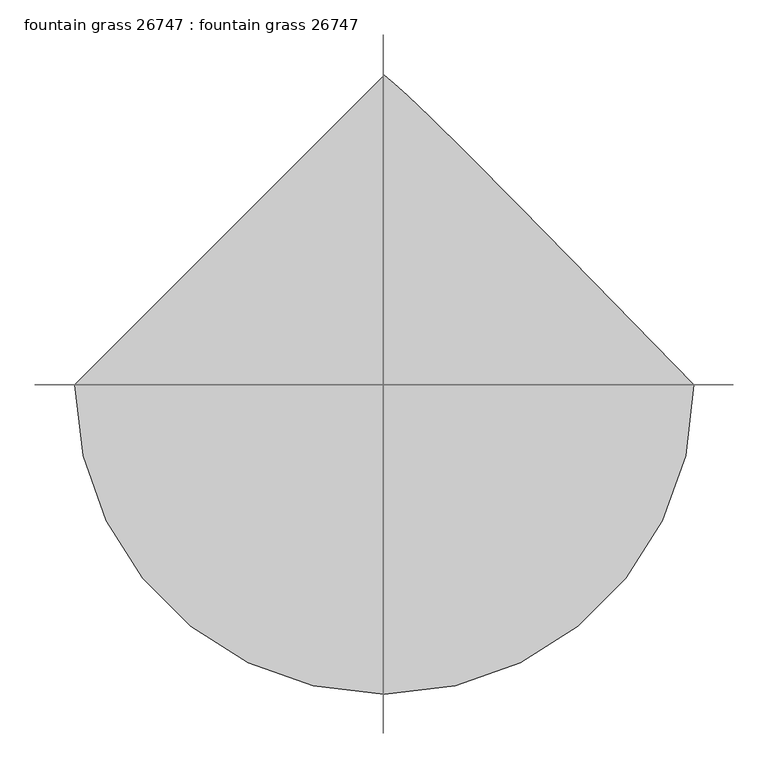
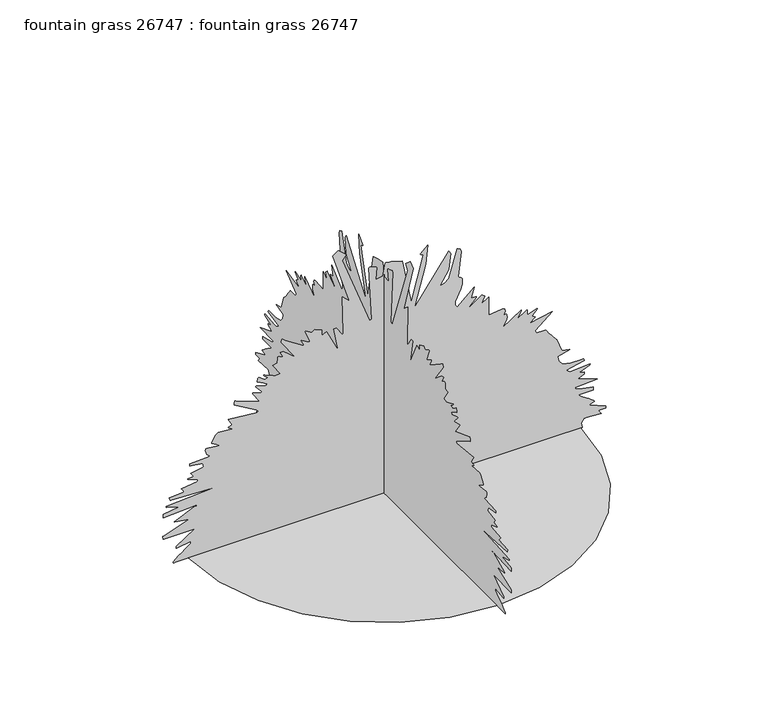
"""IFC4 building model written with IfcOpenShell, lengths in millimetres: proxy geometry, fountain grass 26747 : fountain grass 26747."""

from ifc_helpers import new_model, si_unit, origin, place, context, project, spatial, triangles, source, transform, mapped, element, save


def fountain_grass_26747_fountain_grass_26747_87ae7408(model_context):
    return source(origin(), model_context, "Body", "Tessellation", [
        triangles([(-987.0455658, 0.0, 0.0001807), (-960.952173, -226.1654466, 0.0001807), (-886.6343983, -433.862035, 0.0001807), (-770.0484913, -617.1406734, 0.0001807), (-617.1406734, -770.0484913, 0.0001807), (-433.862035, -886.6343983, 0.0001807), (-226.1654466, -960.952173, 0.0001807), (4.31e-05, -987.0455658, 0.0001807), (226.1657009, -960.952173, 0.0001807), (433.862035, -886.6343983, 0.0001807), (617.1406734, -770.0484913, 0.0001807), (770.0484913, -617.1406734, 0.0001807), (886.6343983, -433.862035, 0.0001807), (960.952173, -226.1654466, 0.0001807), (987.0455658, 8.63e-05, 0.0001807), (666.2769184, 329.0287173, 0.0001807), (428.4772619, 571.2784656, 0.0001807), (259.8137924, 741.2118793, 0.0001807), (146.4631077, 853.2918114, 0.0001807), (74.5956602, 921.9810053, 0.0001807), (30.3837036, 961.7446392, 0.0001807), (-0.0001294, 987.0455658, 0.0001807), (-192.732222, -8.8e-06, 1335.7745705), (-213.2038286, -7.2e-06, 1310.1839813), (-75.0206025, 1.47e-05, 941.6939009), (-74.0421966, 1.47e-05, 941.9784039), (-72.5994794, 1.47e-05, 942.7098999), (-70.8743122, 1.46e-05, 943.7080948), (-69.0480519, 1.45e-05, 944.7977812), (-67.3038361, 1.45e-05, 945.7985195), (-65.8220043, 1.44e-05, 946.5300882), (-64.7846675, 1.44e-05, 946.8119751), (-80.1384406, -2.1e-06, 1223.1789722), (-79.3512975, -2.1e-06, 1223.3695129), (-78.4244554, -2.1e-06, 1223.8850338), (-77.4526488, -2.1e-06, 1224.6394936), (-76.5311389, -2.2e-06, 1225.5436535), (-75.2199908, -2.3e-06, 1227.4587982), (-75.0206025, -2.4e-06, 1228.2971191), (-39.1952093, -1.4e-06, 1212.9427511), (-44.3130519, 2.2e-06, 1151.5281858), (-8.4877319, 1.9e-06, 1156.6462601), (4.7327266, -1.8e-06, 1221.0427654), (6.8660195, -2.1e-06, 1223.1789722), (43.5436857, -1.6e-06, 1215.9958351), (88.7523407, -8e-07, 1202.7066027), (134.8136643, 1.32e-05, 967.2843447), (196.2285203, -5e-07, 1197.5909992), (183.550624, -1e-06, 1203.2526449), (181.3428736, -1.1e-06, 1205.4269308), (180.8747518, -1.1e-06, 1207.8246769), (216.700145, -3.3e-06, 1243.6512691), (206.4644507, 2.5e-06, 1146.4100389), (150.1674419, 1.53e-05, 931.4576797), (324.1773419, -3.2e-06, 1172.2011972), (334.4109833, -2.3e-06, 1156.8469019), (324.1773419, 2.6e-06, 1074.959967), (278.1144741, 6.8e-06, 1003.3091806), (303.186799, 6.4e-06, 1010.2737991), (322.3333048, 5.3e-06, 1028.8183794), (365.1195376, -3.2e-06, 1172.2011972), (380.7405318, -2.8e-06, 1165.3635332), (386.8136713, -1.8e-06, 1149.1050053), (371.0377447, 5.8e-06, 1020.4236883), (372.5033166, 6e-06, 1017.0835579), (375.3150999, 6.2e-06, 1014.6375589), (378.9295232, 6.3e-06, 1012.7299719), (382.8157322, 6.4e-06, 1011.0028244), (386.4301191, 6.5e-06, 1009.0952374), (389.2419024, 6.6e-06, 1006.6492384), (390.7100178, 6.8e-06, 1003.3091806), (390.8116467, 8.5e-06, 974.9780611), (383.7479064, 1e-05, 950.4898756), (355.0433722, 1.34e-05, 892.7557543), (354.7944775, 1.44e-05, 876.299128), (365.1195376, 1.54e-05, 860.0101513), (452.1246194, 1.08e-05, 936.7764685), (436.7703604, 1.39e-05, 885.5980516), (437.4358357, 1.38e-05, 884.2035873), (460.8495229, 1.41e-05, 882.1284233), (462.3608042, 1.42e-05, 880.4799774), (460.8800079, 1.46e-05, 876.8274387), (425.4318083, 1.61e-05, 841.6561117), (426.5341393, 1.66e-05, 839.537709), (430.7911832, 1.6e-05, 840.3353348), (487.9487409, 1.42e-05, 880.4799774), (489.1120783, 1.43e-05, 881.361319), (491.0831062, 1.43e-05, 880.6425402), (503.3030362, 1.48e-05, 870.2437563), (487.9487409, 1.69e-05, 834.4196348), (523.7754058, 1.54e-05, 860.0101513), (523.7754058, 2.12e-05, 762.7688484), (593.7116893, 2.08e-05, 769.8782982), (604.2222033, 2.1e-05, 765.8219324), (607.2778307, 2.16e-05, 755.5679798), (600.5443027, 2.27e-05, 737.1784046), (610.7779804, 2.27e-05, 737.1784046), (611.8422323, 2.27e-05, 736.5230667), (614.1129513, 2.29e-05, 734.0897123), (616.2186367, 2.32e-05, 729.1722799), (616.7773962, 2.37e-05, 721.0722656), (614.4152584, 2.44e-05, 709.086006), (595.4261922, 2.67e-05, 670.6456924), (687.546841, 2.3e-05, 732.0602577), (687.8186268, 2.35e-05, 728.1842588), (667.0770149, 2.55e-05, 691.118062), (716.0887762, 2.38e-05, 722.0933516), (718.2554317, 2.36e-05, 721.8266527), (719.3450455, 2.39e-05, 719.0986942), (717.5061316, 2.5e-05, 697.6534916), (718.2554317, 2.51e-05, 696.2361362), (720.4347319, 2.49e-05, 695.6976517), (766.5382404, 2.45e-05, 712.7029364), (769.4337759, 2.42e-05, 711.5904316), (768.6387663, 2.44e-05, 709.4415802), (744.2522461, 2.59e-05, 683.2440514), (743.8433321, 2.61e-05, 680.8819136), (759.1976274, 2.67e-05, 670.6456924), (728.4915802, 2.82e-05, 645.0577194), (845.0825741, 2.67e-05, 669.6881201), (759.1976274, 3.09e-05, 598.994906), (764.3157017, 3.19e-05, 583.6431541), (810.3760443, 3.19e-05, 583.6431541), (812.6900019, 3.21e-05, 579.4623047), (818.8519804, 3.26e-05, 570.8923699), (827.7013676, 3.33e-05, 559.353176), (838.0696301, 3.41e-05, 546.269636), (848.7985537, 3.49e-05, 533.064192), (858.7223665, 3.56e-05, 521.1643006), (866.6750788, 3.61e-05, 511.9923677), (892.2629791, 4.01e-05, 445.4596919), (933.2077909, 4.07e-05, 435.2234708), (871.793153, 4.16e-05, 419.8692118), (876.9112272, 4.31e-05, 394.2787316), (879.8754358, 4.33e-05, 391.6269676), (882.8904408, 4.35e-05, 388.2919604), (885.7733316, 4.37e-05, 384.6267408), (888.3361839, 4.39e-05, 380.9920063), (890.3960873, 4.41e-05, 377.7407876), (891.7651897, 4.43e-05, 375.2261882), (892.2629791, 4.44e-05, 373.8088692), (895.890156, 4.44e-05, 372.7801892), (938.3258652, 4.5e-05, 363.5726844), (999.7404305, 4.5e-05, 363.5726844), (1000.5278824, 4.5e-05, 362.5440044), (1001.4549334, 4.51e-05, 361.080976), (1002.425223, 4.52e-05, 359.3588428), (1003.3472597, 4.53e-05, 357.5503776), (1004.1219217, 4.54e-05, 355.8282443), (1004.6578629, 4.55e-05, 354.3652159), (1004.8585773, 4.56e-05, 353.3364996), (912.7354214, 4.68e-05, 332.86413), (913.6015022, 4.69e-05, 331.6373154), (915.8976557, 4.7e-05, 329.6383458), (919.1819029, 4.71e-05, 327.1415142), (923.0020912, 4.73e-05, 324.4110123), (926.9110823, 4.75e-05, 321.7160823), (930.4620283, 4.76e-05, 319.3259302), (933.2077909, 4.77e-05, 317.5123781), (949.6695042, 4.77e-05, 318.6757155), (1032.0797356, 4.76e-05, 324.6954789), (1035.5645519, 4.74e-05, 322.6279452), (1033.032221, 4.76e-05, 319.7526484), (979.2680609, 4.89e-05, 297.0400085), (1004.8585773, 4.92e-05, 291.9219162), (1004.8585773, 4.99e-05, 281.6857132), (975.3971489, 5.07e-05, 267.6446189), (974.1499866, 5.08e-05, 266.331436), (1071.3912169, 5.29e-05, 230.5068058), (958.7956913, 5.32e-05, 225.3889678), (958.7956913, 5.35e-05, 220.2708572), (979.2680609, 5.41e-05, 210.0351811), (1050.9188473, 5.5e-05, 194.6814126), (1050.9188473, 5.6e-05, 179.327626), (974.1499866, 5.6e-05, 179.327626), (978.767728, 5.62e-05, 175.5818881), (990.6523224, 5.67e-05, 167.0838239), (1006.8625975, 5.74e-05, 155.6789786), (1024.4520761, 5.81e-05, 143.2134423), (1051.9830992, 5.94e-05, 122.4842661), (1056.0369942, 5.96e-05, 117.9127791), (1055.1428627, 5.97e-05, 116.2480642), (1031.9527084, 6.02e-05, 108.5996212), (1030.4464777, 6.02e-05, 107.6770939), (1112.3334852, 6.24e-05, 71.8517007), (1112.3334852, 6.3e-05, 61.6157658), (1076.5093637, 6.3e-05, 61.6157658), (1088.8461107, 6.4e-05, 43.7974311), (1091.8611156, 6.42e-05, 41.1441501), (1004.8585773, 6.39e-05, 46.2622425), (989.504282, 6.51e-05, 25.7906269), (994.6223562, 6.66e-05, 0.2009925), (-1062.775609, 7.09e-05, 6.89e-05), (-1062.775609, 7.05e-05, 5.1179681), (-1049.4888474, 6.99e-05, 15.7529118), (-1033.944084, 6.92e-05, 27.9602914), (-1017.6728388, 6.84e-05, 40.5703616), (-1002.191589, 6.77e-05, 52.4138656), (-989.0343979, 6.71e-05, 62.3213777), (-979.7176701, 6.67e-05, 69.1234924), (-975.7730707, 6.66e-05, 71.6507864), (-975.7730707, 6.6e-05, 81.8864716), (-1047.4213137, 6.66e-05, 71.6507864), (-1047.4213137, 6.6e-05, 81.8864716), (-955.3006285, 6.23e-05, 143.3013185), (-1113.9564966, 6.23e-05, 143.3013185), (-1114.0479881, 6.22e-05, 144.6553964), (-1114.2638906, 6.21e-05, 147.0447673), (-1114.5102419, 6.19e-05, 150.0158069), (-1114.6931522, 6.17e-05, 153.1156177), (-1114.7261444, 6.16e-05, 155.891066), (-1114.5102419, 6.14e-05, 157.8885276), (-1113.9564966, 6.14e-05, 158.6551051), (-986.0066757, 5.87e-05, 204.7161744), (-1054.7643974, 5.81e-05, 213.3275311), (-1057.6574621, 5.8e-05, 214.9521049), (-955.3006285, 5.53e-05, 261.0126836), (-945.06448, 5.53e-05, 261.0126836), (-945.06448, 5.5e-05, 266.130776), (-1113.9564966, 5.56e-05, 255.8945912), (-1113.9564966, 5.44e-05, 276.3669608), (-1032.0695618, 5.38e-05, 286.6031456), (-1098.6022739, 5.26e-05, 307.0755152), (-1098.6022739, 5.22e-05, 312.1910823), (-852.941324, 5.13e-05, 327.5453776), (-1078.1298317, 5.07e-05, 337.7815624), (-1082.9660191, 4.99e-05, 351.3121319), (-1083.2479786, 4.98e-05, 353.1358578), (-1006.4790453, 4.95e-05, 358.253932), (-1021.1679016, 4.84e-05, 377.3064754), (-1021.8333406, 4.83e-05, 378.7237945), (-939.9464058, 4.77e-05, 388.9599792), (-939.9464058, 4.71e-05, 399.196164), (-983.6648129, 4.62e-05, 414.4208888), (-989.0952953, 4.6e-05, 417.5603411), (-991.1248226, 4.58e-05, 419.6685336), (-960.4187754, 4.55e-05, 424.7866442), (-975.1050156, 4.44e-05, 443.8391513), (-975.7730707, 4.43e-05, 445.2590137), (-909.2403585, 4.37e-05, 455.4926551), (-914.3558893, 4.25e-05, 475.965061), (-980.8911449, 4.19e-05, 486.2012458), (-980.8911449, 4.13e-05, 496.4374306), (-878.5317678, 4.1e-05, 501.5555048), (-879.1134184, 4.09e-05, 503.3716003), (-888.6028828, 4.02e-05, 513.6840159), (-893.8860632, 4e-05, 516.9098001), (-900.7211838, 3.88e-05, 540.5851356), (-900.558621, 3.85e-05, 544.4840255), (-899.0041374, 3.82e-05, 547.6158474), (-894.7090508, 3.84e-05, 548.9721963), (-839.7257063, 3.85e-05, 543.0539892), (-832.4714979, 3.85e-05, 542.4977368), (-834.0945093, 3.85e-05, 545.8555987), (-865.9461262, 3.72e-05, 565.5888419), (-868.2956194, 3.7e-05, 568.088217), (-868.4048424, 3.65e-05, 572.164894), (-848.5039495, 3.46e-05, 604.96896), (-842.4562082, 3.44e-05, 611.1792641), (-837.5895721, 3.42e-05, 614.1485596), (-765.9387857, 3.46e-05, 609.030449), (-780.5183464, 3.41e-05, 617.4352776), (-785.6364206, 3.37e-05, 622.5609821), (-786.4086119, 3.36e-05, 624.384708), (-767.3586119, 3.34e-05, 628.6646067), (-765.9387857, 3.33e-05, 629.5027822), (-786.4086119, 3.12e-05, 665.3269037), (-637.9889648, 3.21e-05, 649.9752245), (-637.7984241, 3.21e-05, 650.9530718), (-637.2828306, 3.2e-05, 652.395789), (-636.5284435, 3.19e-05, 654.1204657), (-635.6242109, 3.18e-05, 655.946735), (-634.6564648, 3.17e-05, 657.6916866), (-633.7090662, 3.16e-05, 659.1725555), (-632.8733614, 3.15e-05, 660.2088295), (-755.7025646, 2.72e-05, 731.8596159), (-755.710195, 2.71e-05, 734.6180958), (-755.6593987, 2.69e-05, 738.1944036), (-755.4384092, 2.67e-05, 742.1339161), (-754.9329895, 2.65e-05, 745.9743793), (-754.0313004, 2.63e-05, 749.26117), (-752.6190319, 2.61e-05, 751.5344324), (-750.5844904, 2.6e-05, 752.3319855), (-627.7552872, 2.88e-05, 706.2717155), (-663.6860882, 2.56e-05, 759.6675116), (-663.5794086, 2.54e-05, 762.5682066), (-660.4755283, 2.56e-05, 763.5054314), (-620.4934484, 2.58e-05, 751.3083561), (-617.5191387, 2.6e-05, 752.3319855), (-618.27854, 2.56e-05, 755.4434961), (-647.6638103, 2.37e-05, 790.1982788), (-648.2251133, 2.36e-05, 793.2742538), (-645.0653498, 2.38e-05, 794.1149729), (-597.0467328, 2.45e-05, 777.9225019), (-596.4675894, 2.44e-05, 778.9130665), (-595.0452198, 2.43e-05, 780.3888485), (-593.2570295, 2.42e-05, 782.1490608), (-591.5755551, 2.41e-05, 784.0032354), (-590.4782747, 2.4e-05, 785.7507305), (-590.4376522, 2.39e-05, 787.201078), (-591.9286222, 2.39e-05, 788.1586504), (-637.9889648, 2.24e-05, 813.7466234), (-639.6145197, 2.21e-05, 815.2045286), (-640.0666723, 2.19e-05, 818.265243), (-638.3851616, 2.15e-05, 826.5253492), (-636.7163681, 2.14e-05, 830.3861601), (-634.8012234, 2.12e-05, 833.1724726), (-632.8733614, 2.11e-05, 834.218993), (-630.4730719, 2.12e-05, 834.2443548), (-602.164807, 2.24e-05, 813.7466234), (-586.810548, 2.2e-05, 818.8646976), (-606.0256179, 2.11e-05, 834.9200403), (-607.7909171, 2.1e-05, 837.6987951), (-607.2829176, 2.08e-05, 839.3370672), (-603.6684943, 2.09e-05, 838.9128925), (-561.8702826, 2.2e-05, 820.0915123), (-550.9864265, 2.24e-05, 813.7466234), (-525.3959464, 2.2e-05, 818.8646976), (-559.8662261, 1.89e-05, 871.7906096), (-561.2226113, 1.87e-05, 875.1611887), (-540.7502054, 1.84e-05, 880.2793356), (-537.9714506, 1.73e-05, 906.7536644), (-536.9859366, 1.7e-05, 909.870262), (-535.6321312, 1.66e-05, 910.9878536), (-533.2191244, 1.68e-05, 912.2654646), (-529.3558064, 1.69e-05, 911.5212513), (-510.0416511, 1.72e-05, 900.7517052), (-525.3959464, 1.53e-05, 931.4576797), (-510.0416511, 1.53e-05, 931.4576797), (-448.6270494, 1.84e-05, 880.2793356), (-520.2778358, 1.23e-05, 982.63864), (-520.4962818, 1.22e-05, 984.7163475), (-516.051277, 1.16e-05, 996.9642191), (-515.2257823, 1.15e-05, 998.3459661), (-515.1597616, 1.14e-05, 997.9903919), (-498.3728866, 1.21e-05, 985.7882298), (-408.0734565, 1.55e-05, 927.9093498), (-402.5667432, 1.56e-05, 926.342149), (-417.4790597, 1.45e-05, 951.9148613), (-418.5687098, 1.42e-05, 955.282897), (-417.9210385, 1.38e-05, 957.0481962), (-415.5080317, 1.41e-05, 957.1853245), (-380.6389392, 1.48e-05, 937.1701944), (-376.976263, 1.5e-05, 936.5758266), (-376.9203798, 1.43e-05, 940.7439589), (-397.9032924, 1.21e-05, 994.048336), (-397.4486326, 1.14e-05, 997.9903919), (-395.0686543, 1.16e-05, 998.5085289), (-366.1584277, 1.23e-05, 982.382115), (-351.3883264, 1.17e-05, 992.8748611), (-315.5616614, 1.26e-05, 977.5205658), (-315.5616614, 1.44e-05, 946.8119751), (-294.1621864, 1.4e-05, 958.3587994), (-291.1294318, 1.39e-05, 958.6407589), (-289.9737247, 1.38e-05, 957.0481962), (-233.6754533, 2.08e-05, 839.3370672), (-254.1470598, 1.35e-05, 962.1662704), (-243.9113837, 1.35e-05, 962.1662704), (-213.2038286, 1.62e-05, 916.1059278), (-211.0877513, 1.6e-05, 916.598703), (-209.5368286, 1.59e-05, 917.6680418), (-208.4642015, 1.57e-05, 919.1971636), (-207.7817031, 1.56e-05, 921.0716858), (-207.4032379, 1.54e-05, 923.1722116), (-207.2399121, 1.53e-05, 925.3845766), (-207.2046126, 1.52e-05, 927.5918547), (-213.2038286, 4.4e-06, 1115.7040644), (-210.5383663, 4.8e-06, 1115.4424524), (-179.2496511, 6.1e-06, 1087.4745375), (-177.3786897, 6.2e-06, 1084.9954737), (-259.2651522, -9.7e-06, 1351.1262497), (-233.6754533, -1.09e-05, 1371.5986919), (-3.3699163, -189.3624059, 1335.7745705), (-3.3699163, -209.8340125, 1310.1839813), (-3.3699163, -71.6505366, 941.6939009), (-3.3699163, -70.6721261, 941.9784039), (-3.3699163, -69.2296633, 942.7098999), (-3.3699163, -67.5042417, 943.7080948), (-3.3699163, -65.6782403, 944.7977812), (-3.3699163, -63.93402, 945.7985195), (-3.3699163, -62.4519338, 946.5300882), (-3.3699163, -61.4148514, 946.8119751), (-3.3699163, -76.7683792, 1223.1789722), (-3.3699163, -75.9812316, 1223.3695129), (-3.3699163, -75.054385, 1223.8850338), (-3.3699163, -74.0828373, 1224.6394936), (-3.3699163, -73.161073, 1225.5436535), (-3.3699163, -71.8499249, 1227.4587982), (-3.3699163, -71.6505366, 1228.2971191), (-3.3699163, -35.8251411, 1212.9427511), (-3.3699163, -40.9429814, 1151.5281858), (-3.3699163, -5.1177648, 1156.6462601), (-3.3699163, 8.1026934, 1221.0427654), (-3.3699163, 10.2359611, 1223.1789722), (-3.3699163, 46.9137516, 1215.9958351), (-3.3699163, 92.122402, 1202.7066027), (-3.3699163, 138.1834804, 967.2843447), (-3.3699163, 199.5985907, 1197.5909992), (-3.3699163, 186.9206945, 1203.2526449), (-3.3699163, 184.7129259, 1205.4269308), (-3.3699163, 184.244804, 1207.8246769), (-3.3699163, 220.0701972, 1243.6512691), (-3.3699163, 209.8342668, 1146.4100389), (-3.3699163, 153.5372671, 931.4576797), (-3.3699163, 327.5453776, 1172.2011972), (-3.3699163, 337.7815624, 1156.8469019), (-3.3699163, 327.5453776, 1074.959967), (-3.3699163, 281.4850532, 1003.3091806), (-3.3699163, 306.5573782, 1010.2737991), (-3.3699163, 325.7038839, 1028.8183794), (-3.3699163, 368.4901168, 1172.2011972), (-3.3699163, 384.1085675, 1165.3635332), (-3.3699163, 390.1842505, 1149.1050053), (-3.3699163, 374.4057804, 1020.4236883), (-3.3699163, 375.8738957, 1017.0835579), (-3.3699163, 378.6856791, 1014.6375589), (-3.3699163, 382.3001023, 1012.7299719), (-3.3699163, 386.1863113, 1011.0028244), (-3.3699163, 389.8006983, 1009.0952374), (-3.3699163, 392.6124816, 1006.6492384), (-3.3699163, 394.0780535, 1003.3091806), (-3.3699163, 394.1796824, 974.9780611), (-3.3699163, 387.1184855, 950.4898756), (-3.3699163, 358.4139513, 892.7557543), (-3.3699163, 358.1650566, 876.299128), (-3.3699163, 368.4901168, 860.0101513), (-3.3699163, 455.4926551, 936.7764685), (-3.3699163, 440.1409032, 885.5980516), (-3.3699163, 440.8038714, 884.2035873), (-3.3699163, 464.2175586, 882.1284233), (-3.3699163, 465.7288399, 880.4799774), (-3.3699163, 464.2505871, 876.8274387), (-3.3699163, 428.8023874, 841.6561117), (-3.3699163, 429.9047184, 839.537709), (-3.3699163, 434.1617623, 840.3353348), (-3.3699163, 491.31932, 880.4799774), (-3.3699163, 492.480114, 881.361319), (-3.3699163, 494.4536854, 880.6425402), (-3.3699163, 506.6736154, 870.2437563), (-3.3699163, 491.31932, 834.4196348), (-3.3699163, 527.1434415, 860.0101513), (-3.3699163, 527.1434415, 762.7688484), (-3.3699163, 597.079725, 769.8782982), (-3.3699163, 607.5927824, 765.8219324), (-3.3699163, 610.6458664, 755.5679798), (-3.3699163, 603.9123384, 737.1784046), (-3.3699163, 614.1485596, 737.1784046), (-3.3699163, 615.2128115, 736.5230667), (-3.3699163, 617.4835304, 734.0897123), (-3.3699163, 619.5866724, 729.1722799), (-3.3699163, 620.1479753, 721.0722656), (-3.3699163, 617.7858376, 709.086006), (-3.3699163, 598.7942279, 670.6456924), (-3.3699163, 690.9174202, 732.0602577), (-3.3699163, 691.1866625, 728.1842588), (-3.3699163, 670.4450506, 691.118062), (-3.3699163, 719.4568119, 722.0933516), (-3.3699163, 721.6260109, 721.8266527), (-3.3699163, 722.7156246, 719.0986942), (-3.3699163, 720.8767107, 697.6534916), (-3.3699163, 721.6260109, 696.2361362), (-3.3699163, 723.805311, 695.6976517), (-3.3699163, 769.9062761, 712.7029364), (-3.3699163, 772.804355, 711.5904316), (-3.3699163, 772.0093454, 709.4415802), (-3.3699163, 747.6202818, 683.2440514), (-3.3699163, 747.2139112, 680.8819136), (-3.3699163, 762.5682066, 670.6456924), (-3.3699163, 731.8596159, 645.0577194), (-3.3699163, 848.4531532, 669.6881201), (-3.3699163, 762.5682066, 598.994906), (-3.3699163, 767.6862808, 583.6431541), (-3.3699163, 813.7466234, 583.6431541), (-3.3699163, 816.0605083, 579.4623047), (-3.3699163, 822.2225595, 570.8923699), (-3.3699163, 831.0694033, 559.353176), (-3.3699163, 841.4402092, 546.269636), (-3.3699163, 852.1691328, 533.064192), (-3.3699163, 862.0904022, 521.1643006), (-3.3699163, 870.0431145, 511.9923677), (-3.3699163, 895.6335583, 445.4596919), (-3.3699163, 936.5758266, 435.2234708), (-3.3699163, 875.1611887, 419.8692118), (-3.3699163, 880.2793356, 394.2787316), (-3.3699163, 883.246015, 391.6269676), (-3.3699163, 886.2610199, 388.289417), (-3.3699163, 889.1439108, 384.6267408), (-3.3699163, 891.7067631, 380.9920063), (-3.3699163, 893.764123, 377.7407876), (-3.3699163, 895.1357689, 375.2261882), (-3.3699163, 895.6335583, 373.8088692), (-3.3699163, 899.2607351, 372.7801892), (-3.3699163, 941.6939009, 363.5726844), (-3.3699163, 1003.1084661, 363.5726844), (-3.3699163, 1003.8959181, 362.5440044), (-3.3699163, 1004.8229691, 361.080976), (-3.3699163, 1005.7958021, 359.3588428), (-3.3699163, 1006.7178389, 357.5503776), (-3.3699163, 1007.4925009, 355.8282443), (-3.3699163, 1008.028442, 354.3652159), (-3.3699163, 1008.226613, 353.3364996), (-3.3699163, 916.1059278, 332.86413), (-3.3699163, 916.9695379, 331.6373154), (-3.3699163, 919.2682348, 329.6383458), (-3.3699163, 922.5499386, 327.1415142), (-3.3699163, 926.3701269, 324.4110123), (-3.3699163, 930.279118, 321.7160823), (-3.3699163, 933.8326075, 319.3259302), (-3.3699163, 936.5758266, 317.5098347), (-3.3699163, 953.0400833, 318.6757155), (-3.3699163, 1035.4503147, 324.6954789), (-3.3699163, 1038.9351311, 322.6279452), (-3.3699163, 1036.4028002, 319.7501049), (-3.3699163, 982.63864, 297.0400085), (-3.3699163, 1008.226613, 291.9219162), (-3.3699163, 1008.226613, 281.6857132), (-3.3699163, 978.767728, 267.6446189), (-3.3699163, 977.5205658, 266.331436), (-3.3699163, 1074.7592525, 230.5068058), (-3.3699163, 962.1662704, 225.3887135), (-3.3699163, 962.1662704, 220.2708572), (-3.3699163, 982.63864, 210.0351811), (-3.3699163, 1054.2894264, 194.6814126), (-3.3699163, 1054.2894264, 179.327626), (-3.3699163, 977.5205658, 179.327626), (-3.3699163, 982.1357637, 175.5818881), (-3.3699163, 994.0229015, 167.0835696), (-3.3699163, 1010.2331766, 155.6787243), (-3.3699163, 1027.8226553, 143.2131879), (-3.3699163, 1055.3536783, 122.4842661), (-3.3699163, 1059.4075733, 117.9127791), (-3.3699163, 1058.5134418, 116.2478099), (-3.3699163, 1035.3207441, 108.5993669), (-3.3699163, 1033.8170568, 107.6768396), (-3.3699163, 1115.7040644, 71.8517007), (-3.3699163, 1115.7040644, 61.6157658), (-3.3699163, 1079.8773994, 61.6157658), (-3.3699163, 1092.2166899, 43.7971768), (-3.3699163, 1095.2316948, 41.1441501), (-3.3699163, 1008.226613, 46.2619882), (-3.3699163, 992.8748611, 25.7903726), (-3.3699163, 997.9929354, 0.2009237), (-3.3699163, -1059.4050299, 0.0), (-3.3699163, -1059.4050299, 5.117917), (-3.3699163, -1046.1182682, 15.7528607), (-3.3699163, -1030.5760483, 27.9600371), (-3.3699163, -1014.3022596, 40.5701072), (-3.3699163, -998.8235533, 52.4138656), (-3.3699163, -985.6638187, 62.3213777), (-3.3699163, -976.3496344, 69.1234924), (-3.3699163, -972.4024916, 71.6507864), (-3.3699163, -972.4024916, 81.8864716), (-3.3699163, -1044.053278, 71.6507864), (-3.3699163, -1044.053278, 81.8864716), (-3.3699163, -951.930122, 143.3013185), (-3.3699163, -1110.5859175, 143.3013185), (-3.3699163, -1110.677409, 144.6553964), (-3.3699163, -1110.8933115, 147.0447673), (-3.3699163, -1111.1396627, 150.0158069), (-3.3699163, -1111.3251165, 153.1156177), (-3.3699163, -1111.3555653, 155.891066), (-3.3699163, -1111.1396627, 157.8885276), (-3.3699163, -1110.5859175, 158.6551051), (-3.3699163, -982.63864, 204.7161744), (-3.3699163, -1051.3938183, 213.3275311), (-3.3699163, -1054.2894264, 214.9521049), (-3.3699163, -951.930122, 261.0126836), (-3.3699163, -941.6939009, 261.0126836), (-3.3699163, -941.6939009, 266.130776), (-3.3699163, -1110.5859175, 255.8945912), (-3.3699163, -1110.5859175, 276.3669608), (-3.3699163, -1028.6989826, 286.6031456), (-3.3699163, -1095.2316948, 307.0755152), (-3.3699163, -1095.2316948, 312.1910823), (-3.3699163, -849.5732883, 327.5453776), (-3.3699163, -1074.7592525, 337.7815624), (-3.3699163, -1079.5954399, 351.3121319), (-3.3699163, -1079.8773994, 353.1358578), (-3.3699163, -1003.1084661, 358.253932), (-3.3699163, -1017.7973225, 377.3064754), (-3.3699163, -1018.4627615, 378.7237945), (-3.3699163, -936.5758266, 388.9599792), (-3.3699163, -936.5758266, 399.196164), (-3.3699163, -980.2942337, 414.4208888), (-3.3699163, -985.7272596, 417.5603411), (-3.3699163, -987.7567869, 419.6685336), (-3.3699163, -957.0481962, 424.7866442), (-3.3699163, -971.7369799, 443.8391513), (-3.3699163, -972.4024916, 445.2590137), (-3.3699163, -905.8697794, 455.4926551), (-3.3699163, -910.9878536, 475.965061), (-3.3699163, -977.5205658, 486.2012458), (-3.3699163, -977.5205658, 496.4374306), (-3.3699163, -875.1611887, 501.5555048), (-3.3699163, -875.7428392, 503.3690932), (-3.3699163, -885.2348471, 513.6814725), (-3.3699163, -890.515484, 516.9098001), (-3.3699163, -897.3506046, 540.5851356), (-3.3699163, -897.1880419, 544.4840255), (-3.3699163, -895.6335583, 547.6158474), (-3.3699163, -891.3384716, 548.9721963), (-3.3699163, -836.3576706, 543.0539892), (-3.3699163, -829.1009188, 542.4977368), (-3.3699163, -830.7239302, 545.8555987), (-3.3699163, -862.5780905, 565.5888419), (-3.3699163, -864.9250402, 568.088217), (-3.3699163, -865.0368067, 572.1623506), (-3.3699163, -845.1333704, 604.96896), (-3.3699163, -839.0856291, 611.1792641), (-3.3699163, -834.218993, 614.1485596), (-3.3699163, -762.5682066, 609.030449), (-3.3699163, -777.1477673, 617.4352776), (-3.3699163, -782.2658415, 622.5609821), (-3.3699163, -783.0405762, 624.384708), (-3.3699163, -763.9880327, 628.6646067), (-3.3699163, -762.5682066, 629.5027822), (-3.3699163, -783.0405762, 665.3269037), (-3.3699163, -634.6209291, 649.9752245), (-3.3699163, -634.427845, 650.9530718), (-3.3699163, -633.9122515, 652.395789), (-3.3699163, -633.1604078, 654.1204657), (-3.3699163, -632.2561752, 655.946735), (-3.3699163, -631.2858856, 657.6916866), (-3.3699163, -630.3410305, 659.1725555), (-3.3699163, -629.5027822, 660.2088295), (-3.3699163, -752.3319855, 731.8596159), (-3.3699163, -752.3396158, 734.6180958), (-3.3699163, -752.291363, 738.1944036), (-3.3699163, -752.0703735, 742.1339161), (-3.3699163, -751.5649538, 745.9743793), (-3.3699163, -750.6632647, 749.26117), (-3.3699163, -749.2484528, 751.5344324), (-3.3699163, -747.2139112, 752.3319855), (-3.3699163, -624.384708, 706.2717155), (-3.3699163, -660.315509, 759.6675116), (-3.3699163, -660.2088295, 762.5682066), (-3.3699163, -657.1049492, 763.5054314), (-3.3699163, -617.1228693, 751.3083561), (-3.3699163, -614.1485596, 752.3319855), (-3.3699163, -614.9079609, 755.4434961), (-3.3699163, -644.2932312, 790.1982788), (-3.3699163, -644.8570776, 793.2742538), (-3.3699163, -641.6947706, 794.1149729), (-3.3699163, -593.6761537, 777.9225019), (-3.3699163, -593.0970102, 778.9130665), (-3.3699163, -591.6771841, 780.3888485), (-3.3699163, -589.8864867, 782.1490608), (-3.3699163, -588.2075194, 784.0032354), (-3.3699163, -587.1076956, 785.7507305), (-3.3699163, -587.0670731, 787.201078), (-3.3699163, -588.5580431, 788.1586504), (-3.3699163, -634.6209291, 813.7466234), (-3.3699163, -636.2439405, 815.2045286), (-3.3699163, -636.6960932, 818.265243), (-3.3699163, -635.0171259, 826.5253492), (-3.3699163, -633.3458616, 830.3861601), (-3.3699163, -631.4306442, 833.1724726), (-3.3699163, -629.5027822, 834.218993), (-3.3699163, -627.1050362, 834.2443548), (-3.3699163, -598.7942279, 813.7466234), (-3.3699163, -583.4399689, 818.8646976), (-3.3699163, -602.6575822, 834.9200403), (-3.3699163, -604.420338, 837.6987951), (-3.3699163, -603.9123384, 839.3370672), (-3.3699163, -600.2979152, 838.9128925), (-3.3699163, -558.5022469, 820.0915123), (-3.3699163, -547.6158474, 813.7466234), (-3.3699163, -522.0253673, 818.8646976), (-3.3699163, -556.495647, 871.7906096), (-3.3699163, -557.8520322, 875.1611887), (-3.3699163, -537.3796263, 880.2793356), (-3.3699163, -534.6008715, 906.7536644), (-3.3699163, -533.6153575, 909.870262), (-3.3699163, -532.261552, 910.9878536), (-3.3699163, -529.8510887, 912.2654646), (-3.3699163, -525.9877707, 911.5212513), (-3.3699163, -506.6736154, 900.7517052), (-3.3699163, -522.0253673, 931.4576797), (-3.3699163, -506.6736154, 931.4576797), (-3.3699163, -445.2564703, 880.2793356), (-3.3699163, -516.9072567, 982.63864), (-3.3699163, -517.1282461, 984.7163475), (-3.3699163, -512.6832413, 996.9642191), (-3.3699163, -511.8552032, 998.3459661), (-3.3699163, -511.7891825, 997.9929354), (-3.3699163, -495.0023074, 985.7882298), (-3.3699163, -404.7028773, 927.9093498), (-3.3699163, -399.196164, 926.342149), (-3.3699163, -414.111024, 951.9148613), (-3.3699163, -415.1981306, 955.282897), (-3.3699163, -414.5504594, 957.0481962), (-3.3699163, -412.1374526, 957.1853245), (-3.3699163, -377.2709035, 937.1701944), (-3.3699163, -373.6056839, 936.5758266), (-3.3699163, -373.5523441, 940.7439589), (-3.3699163, -394.5327132, 994.048336), (-3.3699163, -394.0780535, 997.9929354), (-3.3699163, -391.6980752, 998.5085289), (-3.3699163, -362.790392, 982.382115), (-3.3699163, -348.0177472, 992.8748611), (-3.3699163, -312.1910823, 977.5205658), (-3.3699163, -312.1910823, 946.8119751), (-3.3699163, -290.7916072, 958.3587994), (-3.3699163, -287.7613961, 958.6407589), (-3.3699163, -286.6031456, 957.0481962), (-3.3699163, -230.3056372, 839.3370672), (-3.3699163, -250.7772437, 962.1662704), (-3.3699163, -240.5415676, 962.1662704), (-3.3699163, -209.8340125, 916.1059278), (-3.3699163, -207.7176991, 916.598703), (-3.3699163, -206.1670306, 917.6680418), (-3.3699163, -205.094131, 919.1971636), (-3.3699163, -204.411887, 921.0716858), (-3.3699163, -204.0334218, 923.1722116), (-3.3699163, -203.8698416, 925.3845766), (-3.3699163, -203.8347965, 927.5918547), (-3.3699163, -209.8340125, 1115.7040644), (-3.3699163, -207.1682958, 1115.4424524), (-3.3699163, -175.879835, 1087.4745375), (-3.3699163, -174.0086193, 1084.9954737), (-3.3699163, -255.8945912, 1351.1262497), (-3.3699163, -230.3056372, 1371.5986919)], [[21, 22, 1], [20, 21, 1], [19, 20, 1], [18, 19, 1], [17, 18, 1], [17, 1, 2], [17, 2, 3], [17, 3, 4], [16, 17, 4], [16, 4, 5], [16, 5, 6], [16, 6, 7], [16, 7, 8], [16, 8, 9], [16, 9, 10], [16, 10, 11], [16, 11, 12], [15, 16, 12], [14, 15, 12], [13, 14, 12], [168, 169, 170], [119, 120, 121], [131, 132, 133], [76, 77, 78], [188, 189, 190], [333, 334, 335], [215, 216, 217], [266, 267, 268], [90, 91, 92], [235, 236, 237], [234, 235, 237], [214, 215, 217], [103, 104, 105], [103, 105, 106], [327, 328, 329], [233, 234, 237], [54, 55, 56], [54, 56, 57], [54, 57, 58], [230, 231, 232], [117, 118, 119], [238, 239, 240], [229, 230, 232], [60, 61, 62], [60, 62, 63], [191, 192, 193], [161, 162, 163], [38, 39, 40], [356, 357, 358], [356, 358, 359], [237, 238, 240], [202, 203, 204], [202, 204, 205], [187, 188, 190], [319, 320, 321], [366, 367, 368], [366, 368, 369], [366, 369, 370], [227, 228, 229], [219, 220, 221], [219, 221, 222], [191, 193, 194], [191, 194, 195], [191, 195, 196], [191, 196, 197], [191, 197, 198], [191, 198, 199], [191, 199, 200], [191, 200, 201], [185, 186, 187], [184, 185, 187], [184, 187, 190], [173, 174, 175], [172, 173, 175], [113, 114, 115], [191, 201, 202], [191, 202, 205], [226, 227, 229], [225, 226, 229], [225, 229, 232], [150, 151, 152], [149, 150, 152], [148, 149, 152], [147, 148, 152], [146, 147, 152], [145, 146, 152], [144, 145, 152], [143, 144, 152], [372, 23, 24], [371, 372, 24], [370, 371, 24], [370, 24, 25], [366, 370, 25], [242, 243, 244], [241, 242, 244], [223, 224, 225], [222, 223, 225], [219, 222, 225], [205, 206, 207], [291, 292, 293], [333, 335, 336], [205, 207, 208], [76, 78, 79], [205, 208, 209], [205, 209, 210], [205, 210, 211], [205, 211, 212], [205, 212, 213], [205, 213, 214], [332, 333, 336], [331, 332, 336], [330, 331, 336], [330, 336, 337], [365, 366, 25], [37, 38, 40], [60, 63, 64], [262, 263, 264], [32, 33, 34], [313, 314, 315], [312, 313, 315], [311, 312, 315], [364, 365, 25], [164, 165, 166], [160, 161, 163], [160, 163, 164], [318, 319, 321], [37, 40, 41], [36, 37, 41], [35, 36, 41], [34, 35, 41], [32, 34, 41], [32, 41, 42], [112, 113, 115], [112, 115, 116], [171, 172, 175], [363, 364, 25], [262, 264, 265], [261, 262, 265], [346, 347, 348], [346, 348, 349], [285, 286, 287], [290, 291, 293], [290, 293, 294], [180, 181, 182], [233, 237, 240], [350, 351, 352], [340, 341, 342], [339, 340, 342], [338, 339, 342], [338, 342, 343], [284, 285, 287], [284, 287, 288], [179, 180, 182], [179, 182, 183], [179, 183, 184], [330, 337, 338], [80, 81, 82], [79, 80, 82], [76, 79, 82], [76, 82, 83], [261, 265, 266], [261, 266, 268], [356, 359, 360], [214, 217, 218], [205, 214, 218], [191, 205, 218], [191, 218, 219], [191, 219, 225], [190, 191, 225], [184, 190, 225], [179, 184, 225], [178, 179, 225], [177, 178, 225], [176, 177, 225], [175, 176, 225], [171, 175, 225], [170, 171, 225], [168, 170, 225], [107, 108, 109], [106, 107, 109], [106, 109, 110], [362, 363, 25], [122, 123, 124], [142, 143, 152], [112, 116, 117], [112, 117, 119], [111, 112, 119], [130, 131, 133], [275, 276, 277], [275, 277, 278], [275, 278, 279], [275, 279, 280], [275, 280, 281], [275, 281, 282], [275, 282, 283], [275, 283, 284], [353, 354, 355], [349, 350, 352], [346, 349, 352], [345, 346, 352], [344, 345, 352], [86, 87, 88], [289, 290, 294], [60, 64, 65], [59, 60, 65], [50, 51, 52], [49, 50, 52], [48, 49, 52], [48, 52, 53], [47, 48, 53], [47, 53, 54], [284, 288, 289], [164, 166, 167], [160, 164, 167], [160, 167, 168], [159, 160, 168], [159, 168, 225], [158, 159, 225], [157, 158, 225], [156, 157, 225], [155, 156, 225], [154, 155, 225], [153, 154, 225], [152, 153, 225], [142, 152, 225], [141, 142, 225], [140, 141, 225], [139, 140, 225], [138, 139, 225], [137, 138, 225], [136, 137, 225], [135, 136, 225], [134, 135, 225], [133, 134, 225], [130, 133, 225], [129, 130, 225], [128, 129, 225], [127, 128, 225], [126, 127, 225], [125, 126, 225], [124, 125, 225], [122, 124, 225], [121, 122, 225], [119, 121, 225], [111, 119, 225], [110, 111, 225], [225, 232, 233], [225, 233, 240], [43, 44, 45], [93, 94, 95], [93, 95, 96], [92, 93, 96], [311, 315, 316], [42, 43, 45], [42, 45, 46], [32, 42, 46], [32, 46, 47], [32, 47, 54], [353, 355, 356], [352, 353, 356], [344, 352, 356], [59, 65, 66], [249, 250, 251], [248, 249, 251], [247, 248, 251], [246, 247, 251], [245, 246, 251], [245, 251, 252], [244, 245, 252], [244, 252, 253], [327, 329, 330], [76, 83, 84], [361, 362, 25], [240, 241, 244], [225, 240, 244], [225, 244, 253], [255, 256, 257], [254, 255, 257], [254, 257, 258], [254, 258, 259], [254, 259, 260], [254, 260, 261], [253, 254, 261], [302, 303, 304], [225, 253, 261], [225, 261, 268], [356, 360, 361], [356, 361, 25], [86, 88, 89], [85, 86, 89], [85, 89, 90], [85, 90, 92], [84, 85, 92], [324, 325, 326], [301, 302, 304], [301, 304, 305], [301, 305, 306], [301, 306, 307], [301, 307, 308], [301, 308, 309], [301, 309, 310], [301, 310, 311], [301, 311, 316], [300, 301, 316], [300, 316, 317], [299, 300, 317], [338, 343, 344], [338, 344, 356], [330, 338, 356], [323, 324, 326], [322, 323, 326], [322, 326, 327], [321, 322, 327], [318, 321, 327], [318, 327, 330], [318, 330, 356], [96, 97, 98], [96, 98, 99], [96, 99, 100], [96, 100, 101], [96, 101, 102], [92, 96, 102], [92, 102, 103], [59, 66, 67], [284, 289, 294], [59, 67, 68], [59, 68, 69], [59, 69, 70], [59, 70, 71], [59, 71, 72], [59, 72, 73], [58, 59, 73], [54, 58, 73], [54, 73, 74], [54, 74, 75], [54, 75, 76], [299, 317, 318], [298, 299, 318], [298, 318, 356], [297, 298, 356], [296, 297, 356], [295, 296, 356], [294, 295, 356], [284, 294, 356], [275, 284, 356], [274, 275, 356], [273, 274, 356], [272, 273, 356], [271, 272, 356], [270, 271, 356], [269, 270, 356], [268, 269, 356], [225, 268, 356], [76, 84, 92], [76, 92, 103], [54, 76, 103], [32, 54, 103], [31, 32, 103], [30, 31, 103], [29, 30, 103], [28, 29, 103], [27, 28, 103], [26, 27, 103], [25, 26, 103], [356, 25, 103], [225, 356, 103], [110, 225, 103], [110, 103, 106], [518, 519, 520], [469, 470, 471], [481, 482, 483], [426, 427, 428], [538, 539, 540], [683, 684, 685], [565, 566, 567], [616, 617, 618], [440, 441, 442], [585, 586, 587], [584, 585, 587], [564, 565, 567], [453, 454, 455], [453, 455, 456], [677, 678, 679], [583, 584, 587], [404, 405, 406], [404, 406, 407], [404, 407, 408], [580, 581, 582], [467, 468, 469], [588, 589, 590], [579, 580, 582], [410, 411, 412], [410, 412, 413], [541, 542, 543], [511, 512, 513], [388, 389, 390], [706, 707, 708], [706, 708, 709], [587, 588, 590], [552, 553, 554], [552, 554, 555], [537, 538, 540], [669, 670, 671], [716, 717, 718], [716, 718, 719], [716, 719, 720], [577, 578, 579], [569, 570, 571], [569, 571, 572], [541, 543, 544], [541, 544, 545], [541, 545, 546], [541, 546, 547], [541, 547, 548], [541, 548, 549], [541, 549, 550], [541, 550, 551], [535, 536, 537], [534, 535, 537], [534, 537, 540], [523, 524, 525], [522, 523, 525], [463, 464, 465], [541, 551, 552], [541, 552, 555], [576, 577, 579], [575, 576, 579], [575, 579, 582], [500, 501, 502], [499, 500, 502], [498, 499, 502], [497, 498, 502], [496, 497, 502], [495, 496, 502], [494, 495, 502], [493, 494, 502], [722, 373, 374], [721, 722, 374], [720, 721, 374], [720, 374, 375], [716, 720, 375], [592, 593, 594], [591, 592, 594], [573, 574, 575], [572, 573, 575], [569, 572, 575], [555, 556, 557], [641, 642, 643], [683, 685, 686], [555, 557, 558], [426, 428, 429], [555, 558, 559], [555, 559, 560], [555, 560, 561], [555, 561, 562], [555, 562, 563], [555, 563, 564], [682, 683, 686], [681, 682, 686], [680, 681, 686], [680, 686, 687], [715, 716, 375], [387, 388, 390], [410, 413, 414], [612, 613, 614], [382, 383, 384], [663, 664, 665], [662, 663, 665], [661, 662, 665], [714, 715, 375], [514, 515, 516], [510, 511, 513], [510, 513, 514], [668, 669, 671], [387, 390, 391], [386, 387, 391], [385, 386, 391], [384, 385, 391], [382, 384, 391], [382, 391, 392], [462, 463, 465], [462, 465, 466], [521, 522, 525], [713, 714, 375], [612, 614, 615], [611, 612, 615], [696, 697, 698], [696, 698, 699], [635, 636, 637], [640, 641, 643], [640, 643, 644], [530, 531, 532], [583, 587, 590], [700, 701, 702], [690, 691, 692], [689, 690, 692], [688, 689, 692], [688, 692, 693], [634, 635, 637], [634, 637, 638], [529, 530, 532], [529, 532, 533], [529, 533, 534], [680, 687, 688], [430, 431, 432], [429, 430, 432], [426, 429, 432], [426, 432, 433], [611, 615, 616], [611, 616, 618], [706, 709, 710], [564, 567, 568], [555, 564, 568], [541, 555, 568], [541, 568, 569], [541, 569, 575], [540, 541, 575], [534, 540, 575], [529, 534, 575], [528, 529, 575], [527, 528, 575], [526, 527, 575], [525, 526, 575], [521, 525, 575], [520, 521, 575], [518, 520, 575], [457, 458, 459], [456, 457, 459], [456, 459, 460], [712, 713, 375], [472, 473, 474], [492, 493, 502], [462, 466, 467], [462, 467, 469], [461, 462, 469], [480, 481, 483], [625, 626, 627], [625, 627, 628], [625, 628, 629], [625, 629, 630], [625, 630, 631], [625, 631, 632], [625, 632, 633], [625, 633, 634], [703, 704, 705], [699, 700, 702], [696, 699, 702], [695, 696, 702], [694, 695, 702], [436, 437, 438], [639, 640, 644], [410, 414, 415], [409, 410, 415], [400, 401, 402], [399, 400, 402], [398, 399, 402], [398, 402, 403], [397, 398, 403], [397, 403, 404], [634, 638, 639], [514, 516, 517], [510, 514, 517], [510, 517, 518], [509, 510, 518], [509, 518, 575], [508, 509, 575], [507, 508, 575], [506, 507, 575], [505, 506, 575], [504, 505, 575], [503, 504, 575], [502, 503, 575], [492, 502, 575], [491, 492, 575], [490, 491, 575], [489, 490, 575], [488, 489, 575], [487, 488, 575], [486, 487, 575], [485, 486, 575], [484, 485, 575], [483, 484, 575], [480, 483, 575], [479, 480, 575], [478, 479, 575], [477, 478, 575], [476, 477, 575], [475, 476, 575], [474, 475, 575], [472, 474, 575], [471, 472, 575], [469, 471, 575], [461, 469, 575], [460, 461, 575], [575, 582, 583], [575, 583, 590], [393, 394, 395], [443, 444, 445], [443, 445, 446], [442, 443, 446], [661, 665, 666], [392, 393, 395], [392, 395, 396], [382, 392, 396], [382, 396, 397], [382, 397, 404], [703, 705, 706], [702, 703, 706], [694, 702, 706], [409, 415, 416], [599, 600, 601], [598, 599, 601], [597, 598, 601], [596, 597, 601], [595, 596, 601], [595, 601, 602], [594, 595, 602], [594, 602, 603], [677, 679, 680], [426, 433, 434], [711, 712, 375], [590, 591, 594], [575, 590, 594], [575, 594, 603], [605, 606, 607], [604, 605, 607], [604, 607, 608], [604, 608, 609], [604, 609, 610], [604, 610, 611], [603, 604, 611], [652, 653, 654], [575, 603, 611], [575, 611, 618], [706, 710, 711], [706, 711, 375], [436, 438, 439], [435, 436, 439], [435, 439, 440], [435, 440, 442], [434, 435, 442], [674, 675, 676], [651, 652, 654], [651, 654, 655], [651, 655, 656], [651, 656, 657], [651, 657, 658], [651, 658, 659], [651, 659, 660], [651, 660, 661], [651, 661, 666], [650, 651, 666], [650, 666, 667], [649, 650, 667], [688, 693, 694], [688, 694, 706], [680, 688, 706], [673, 674, 676], [672, 673, 676], [672, 676, 677], [671, 672, 677], [668, 671, 677], [668, 677, 680], [668, 680, 706], [446, 447, 448], [446, 448, 449], [446, 449, 450], [446, 450, 451], [446, 451, 452], [442, 446, 452], [442, 452, 453], [409, 416, 417], [634, 639, 644], [409, 417, 418], [409, 418, 419], [409, 419, 420], [409, 420, 421], [409, 421, 422], [409, 422, 423], [408, 409, 423], [404, 408, 423], [404, 423, 424], [404, 424, 425], [404, 425, 426], [649, 667, 668], [648, 649, 668], [648, 668, 706], [647, 648, 706], [646, 647, 706], [645, 646, 706], [644, 645, 706], [634, 644, 706], [625, 634, 706], [624, 625, 706], [623, 624, 706], [622, 623, 706], [621, 622, 706], [620, 621, 706], [619, 620, 706], [618, 619, 706], [575, 618, 706], [426, 434, 442], [426, 442, 453], [404, 426, 453], [382, 404, 453], [381, 382, 453], [380, 381, 453], [379, 380, 453], [378, 379, 453], [377, 378, 453], [376, 377, 453], [375, 376, 453], [706, 375, 453], [575, 706, 453], [460, 575, 453], [460, 453, 456]], closed=False),
    ])


if __name__ == "__main__":
    model = new_model("IFC4")
    model_context = context("Model", 3, world=origin())
    ifc_project = project(units=[si_unit("LENGTHUNIT", "METRE", prefix="MILLI")], contexts=[model_context])
    site = spatial("IfcSite", under=ifc_project)
    building = spatial("IfcBuilding", under=site)
    placement = place(None, origin())
    fountain_grass_26747_fountain_grass_26747_shape = fountain_grass_26747_fountain_grass_26747_87ae7408(model_context)
    element("IfcBuildingElementProxy", 1, Name="fountain grass 26747 : fountain grass 26747", ObjectType="fountain grass 26747 : fountain grass 26747", at=placement, inside=building, context=model_context, shape_type="MappedRepresentation", body=[
        mapped(fountain_grass_26747_fountain_grass_26747_shape, transform((0.0, 0.0, 0.0), x_axis=(1.0, 0.0, 0.0), y_axis=(0.0, 1.0, 0.0), z_axis=(0.0, 0.0, 1.0))),
    ])
    save(model, "model.ifc")

# Revit data of these elements
# Type "fountain grass 26747 : fountain grass 26747"
#   built-in parameter 1005195 = "RPC-16-FXGG-QKFX-PG74-4000-ST1L-LVER-AU"
#   Height = 0
